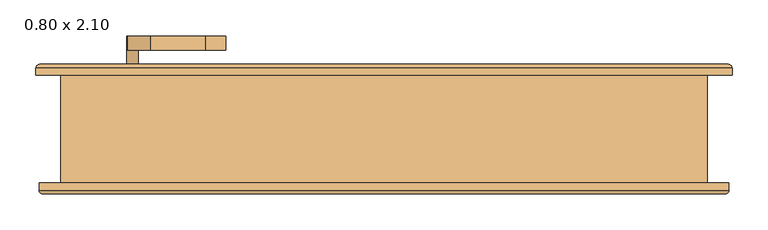
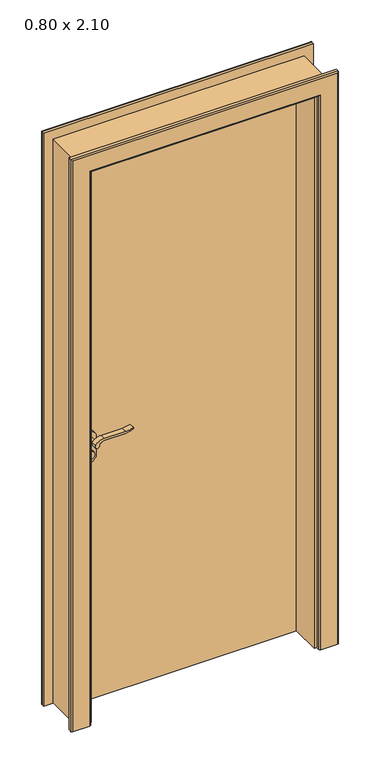
"""IFC4 building model written with IfcOpenShell, lengths in millimetres: door geometry, PORTA_DE_ABRIR_MADEIRA : 0.80 x 2.10."""

from ifc_helpers import new_model, si_unit, point, frame, frame_2d, origin, origin_with_axes, place, context, project, spatial, polyline, circle_curve, ellipse_curve, trimmed, segment, composite_curve, outline, extrude, faceted_brep, source, transform, mapped, element, save
from ifc_brep_helpers import plane_surface, cylinder_surface, advanced_brep


def door_0_80_x_2_10_1ca43dfd(model_context):
    return source(origin(), model_context, "Body", "SolidModel", [
        extrude(outline(composite_curve([segment(trimmed(circle_curve(frame_2d((940.0, -350.0)), 15.0), [point((940.0, -335.0))], [point((940.0, -365.0))], False, "CARTESIAN"), True, "CONTINUOUS"), segment(trimmed(circle_curve(frame_2d((940.0, -350.0)), 15.0), [point((940.0, -365.0))], [point((940.0, -335.0))], False, "CARTESIAN"), True, "CONTINUOUS")], self_intersect=False)), frame((0.0, 15.0, 0.0), z_axis=(0.0, 1.0, 0.0), x_axis=(0.0, 0.0, 1.0)), (0.0, 0.0, 1.0), 10.0),
        extrude(outline(composite_curve([segment(trimmed(circle_curve(frame_2d((940.0, -350.0)), 15.0), [point((940.0, -335.0))], [point((940.0, -365.0))], False, "CARTESIAN"), True, "CONTINUOUS"), segment(trimmed(circle_curve(frame_2d((940.0, -350.0)), 15.0), [point((940.0, -365.0))], [point((940.0, -335.0))], False, "CARTESIAN"), True, "CONTINUOUS")], self_intersect=False)), frame((0.0, 80.0, 0.0), z_axis=(0.0, 1.0, 0.0), x_axis=(0.0, 0.0, 1.0)), (0.0, 0.0, 1.0), 10.0),
        extrude(outline(composite_curve([segment(trimmed(circle_curve(frame_2d((1000.0, -350.0)), 8.0), [point((1004.6523287, -356.5081363))], [point((1000.0, -342.0))], False, "CARTESIAN"), True, "CONTINUOUS"), segment(trimmed(circle_curve(frame_2d((994.8738613, -324.6138099)), 18.1261387), [point((1000.0, -342.0))], [point((1013.0, -324.6138099))], True, "CARTESIAN"), True, "CONTINUOUS"), segment(polyline([(1013.0, -324.6138099), (1013.0, -248.3564091)]), True, "CONTINUOUS"), segment(trimmed(circle_curve(frame_2d((1072.2709207, -251.9396612)), 59.3791355), [point((1013.0, -248.3564091))], [point((1022.2135558, -220.0))], False, "CARTESIAN"), True, "CONTINUOUS"), segment(polyline([(1022.2135558, -220.0), (1025.0, -220.0)]), True, "CONTINUOUS"), segment(trimmed(circle_curve(frame_2d((1103.2850638, -248.4227909)), 83.2850902), [point((1025.0, -220.0))], [point((1020.0, -248.3564091))], True, "CARTESIAN"), True, "CONTINUOUS"), segment(polyline([(1020.0, -248.3564091), (1020.0, -324.6325667)]), True, "CONTINUOUS"), segment(trimmed(circle_curve(frame_2d((982.7555521, -326.3324871)), 37.2832219), [point((1020.0, -324.6325667))], [point((1004.6523287, -356.5081363))], False, "CARTESIAN"), True, "CONTINUOUS")], self_intersect=False)), frame((0.0, -25.0, 0.0), z_axis=(0.0, 1.0, 0.0), x_axis=(0.0, 0.0, 1.0)), (0.0, 0.0, 1.0), 20.0),
        extrude(outline(composite_curve([segment(trimmed(circle_curve(frame_2d((994.8738682, -324.6138122)), 18.1261318), [point((999.9999903, -342.0))], [point((1013.0, -324.6138122))], True, "CARTESIAN"), True, "CONTINUOUS"), segment(polyline([(1013.0, -324.6138122), (1013.0, -248.3564091)]), True, "CONTINUOUS"), segment(trimmed(circle_curve(frame_2d((1072.2709207, -251.9396612)), 59.3791355), [point((1013.0, -248.3564091))], [point((1022.2135558, -220.0))], False, "CARTESIAN"), True, "CONTINUOUS"), segment(polyline([(1022.2135558, -220.0), (1025.0, -220.0)]), True, "CONTINUOUS"), segment(trimmed(circle_curve(frame_2d((1103.2850638, -248.4227909)), 83.2850902), [point((1025.0, -220.0))], [point((1020.0, -248.3564091))], True, "CARTESIAN"), True, "CONTINUOUS"), segment(polyline([(1020.0, -248.3564091), (1020.0, -324.6325667)]), True, "CONTINUOUS"), segment(trimmed(circle_curve(frame_2d((982.7555521, -326.3324871)), 37.2832219), [point((1020.0, -324.6325667))], [point((1004.6523287, -356.5081363))], False, "CARTESIAN"), True, "CONTINUOUS"), segment(trimmed(circle_curve(frame_2d((1000.0, -350.0)), 8.0), [point((1004.6523287, -356.5081363))], [point((999.9999903, -342.0))], False, "CARTESIAN"), True, "CONTINUOUS")], self_intersect=False)), frame((0.0, 110.0, 0.0), z_axis=(0.0, 1.0, 0.0), x_axis=(0.0, 0.0, 1.0)), (0.0, 0.0, 1.0), 20.0),
        extrude(outline(composite_curve([segment(trimmed(circle_curve(frame_2d((1000.0, -350.0)), 8.0), [point((1000.0, -342.0))], [point((1000.0, -358.0))], False, "CARTESIAN"), True, "CONTINUOUS"), segment(trimmed(circle_curve(frame_2d((1000.0, -350.0)), 8.0), [point((1000.0, -358.0))], [point((1000.0, -342.0))], False, "CARTESIAN"), True, "CONTINUOUS")], self_intersect=False)), frame((0.0, -5.0, 0.0), z_axis=(0.0, 1.0, 0.0), x_axis=(0.0, 0.0, 1.0)), (0.0, 0.0, 1.0), 30.0),
        extrude(outline(composite_curve([segment(trimmed(circle_curve(frame_2d((1000.0, -350.0)), 8.0), [point((1000.0, -342.0))], [point((1000.0, -358.0))], False, "CARTESIAN"), True, "CONTINUOUS"), segment(trimmed(circle_curve(frame_2d((1000.0, -350.0)), 8.0), [point((1000.0, -358.0))], [point((1000.0, -342.0))], False, "CARTESIAN"), True, "CONTINUOUS")], self_intersect=False)), frame((0.0, 80.0, 0.0), z_axis=(0.0, 1.0, 0.0), x_axis=(0.0, 0.0, 1.0)), (0.0, 0.0, 1.0), 30.0),
        extrude(outline(composite_curve([segment(trimmed(circle_curve(frame_2d((930.0, -350.0)), 25.0), [point((930.0, -375.0))], [point((930.0, -325.0))], False, "CARTESIAN"), True, "CONTINUOUS"), segment(polyline([(930.0, -325.0), (1000.0, -325.0)]), True, "CONTINUOUS"), segment(trimmed(circle_curve(frame_2d((1000.0, -350.0)), 25.0), [point((1000.0, -325.0))], [point((1000.0, -375.0))], False, "CARTESIAN"), True, "CONTINUOUS"), segment(polyline([(1000.0, -375.0), (930.0, -375.0)]), True, "CONTINUOUS")], self_intersect=False)), frame((0.0, 25.0, 0.0), z_axis=(0.0, 1.0, 0.0), x_axis=(0.0, 0.0, 1.0)), (0.0, 0.0, 1.0), 10.0),
        extrude(outline(composite_curve([segment(trimmed(circle_curve(frame_2d((930.0, -350.0)), 25.0), [point((930.0, -375.0))], [point((930.0, -325.0))], False, "CARTESIAN"), True, "CONTINUOUS"), segment(polyline([(930.0, -325.0), (1000.0, -325.0)]), True, "CONTINUOUS"), segment(trimmed(circle_curve(frame_2d((1000.0, -350.0)), 25.0), [point((1000.0, -325.0))], [point((1000.0, -375.0))], False, "CARTESIAN"), True, "CONTINUOUS"), segment(polyline([(1000.0, -375.0), (930.0, -375.0)]), True, "CONTINUOUS")], self_intersect=False)), frame((0.0, 70.0, 0.0), z_axis=(0.0, 1.0, 0.0), x_axis=(0.0, 0.0, 1.0)), (0.0, 0.0, 1.0), 10.0),
        faceted_brep([(-410.0, 35.0, 0.0), (-400.0, 35.0, 0.0), (-400.0, -75.0, 0.0), (-450.0, -75.0, 0.0), (-450.0, 75.0, 0.0), (-410.0, 75.0, 0.0), (-410.0, 75.0, 2100.0), (-410.0, 35.0, 2100.0), (-450.0, 75.0, 2140.0), (450.0, 75.0, 2140.0), (450.0, 75.0, 0.0), (410.0, 75.0, 0.0), (410.0, 75.0, 2100.0), (-450.0, -75.0, 2140.0), (-400.0, -75.0, 2090.0), (400.0, -75.0, 2090.0), (400.0, -75.0, 0.0), (450.0, -75.0, 0.0), (450.0, -75.0, 2140.0), (-400.0, 35.0, 2090.0), (410.0, 35.0, 2100.0), (410.0, 35.0, 0.0), (400.0, 35.0, 0.0), (400.0, 35.0, 2090.0)], [[[0, 1, 2, 3, 4, 5]], [[5, 6, 7, 0]], [[4, 8, 9, 10, 11, 12, 6, 5]], [[3, 13, 8, 4]], [[2, 14, 15, 16, 17, 18, 13, 3]], [[1, 19, 14, 2]], [[0, 7, 20, 21, 22, 23, 19, 1]], [[23, 22, 16, 15]], [[21, 11, 10, 17, 16, 22]], [[12, 11, 21, 20]], [[18, 17, 10, 9]], [[13, 18, 9, 8]], [[19, 23, 15, 14]], [[6, 12, 20, 7]]]),
        advanced_brep(
        [(-480.0, -75.3, 0.0), (-410.0, -75.3, 0.0), (-410.0, -85.3, 0.0), (-415.0, -90.3, 0.0), (-475.0, -90.3, 0.0), (-480.0, -85.3, 0.0), (-480.0, -85.3, 2170.0), (-480.0, -75.3, 2170.0), (-475.0, -90.3, 2165.0), (-415.0, -90.3, 2105.0), (415.0, -90.3, 2105.0), (415.0, -90.3, 0.0), (475.0, -90.3, 0.0), (475.0, -90.3, 2165.0), (-410.0, -85.3, 2100.0), (-410.0, -75.3, 2100.0), (480.0, -75.3, 2170.0), (480.0, -75.3, 0.0), (410.0, -75.3, 0.0), (410.0, -75.3, 2100.0), (480.0, -85.3, 0.0), (410.0, -85.3, 0.0), (410.0, -85.3, 2100.0), (480.0, -85.3, 2170.0)],
        [
            (0, 1),
            (1, 2),
            (2, 3, circle_curve(frame((-415.0, -85.3, 0.0), z_axis=(0.0, 0.0, -1.0), x_axis=(-1.0, 0.0, 0.0)), 5.0)),
            (3, 4),
            (4, 5, circle_curve(frame((-475.0, -85.3, 0.0), z_axis=(0.0, 0.0, -1.0), x_axis=(-1.0, 0.0, 0.0)), 5.0)),
            (5, 0),
            (5, 6),
            (6, 7),
            (7, 0),
            (4, 8),
            (8, 6, ellipse_curve(frame((-475.0, -85.3, 2165.0), z_axis=(-0.7071067811865475, 0.0, -0.7071067811865475), x_axis=(0.7071067811865474, 0.0, -0.7071067811865476)), 7.0710678, 5.0)),
            (3, 9),
            (9, 10),
            (10, 11),
            (11, 12),
            (12, 13),
            (13, 8),
            (2, 14),
            (14, 9, ellipse_curve(frame((-415.0, -85.3, 2105.0), z_axis=(-0.7071067811865475, 0.0, -0.7071067811865475), x_axis=(0.7071067811865474, 0.0, -0.7071067811865476)), 7.0710678, 5.0)),
            (1, 15),
            (15, 14),
            (7, 16),
            (16, 17),
            (17, 18),
            (18, 19),
            (19, 15),
            (17, 20),
            (20, 12, circle_curve(frame((475.0, -85.3, 0.0), z_axis=(0.0, 0.0, -1.0), x_axis=(1.0, 0.0, 0.0)), 5.0)),
            (11, 21, circle_curve(frame((415.0, -85.3, 0.0), z_axis=(0.0, 0.0, -1.0), x_axis=(1.0, 0.0, 0.0)), 5.0)),
            (21, 18),
            (21, 22),
            (22, 19),
            (10, 22, ellipse_curve(frame((415.0, -85.3, 2105.0), z_axis=(0.7071067811865475, 0.0, -0.7071067811865475), x_axis=(0.7071067811865474, 0.0, 0.7071067811865476)), 7.0710678, 5.0)),
            (20, 23),
            (23, 13, ellipse_curve(frame((475.0, -85.3, 2165.0), z_axis=(0.7071067811865475, 0.0, -0.7071067811865475), x_axis=(0.7071067811865474, 0.0, 0.7071067811865476)), 7.0710678, 5.0)),
            (16, 23),
            (6, 23),
            (22, 14),
        ],
        [
            plane_surface(frame((-450.0, 75.0, 0.0), z_axis=(0.0, 0.0, -1.0), x_axis=(0.0, 1.0, 0.0))),
            plane_surface(frame((-480.0, -75.3, 0.0), z_axis=(-1.0, 0.0, 0.0), x_axis=(0.0, 0.0, 1.0))),
            cylinder_surface(frame((-475.0, -85.3, 0.0), z_axis=(0.0, 0.0, -1.0), x_axis=(-1.0, 0.0, 0.0)), 5.0),
            plane_surface(frame((-475.0, -90.3, 0.0), z_axis=(0.0, -1.0, 0.0), x_axis=(0.0, 0.0, 1.0))),
            cylinder_surface(frame((-415.0, -85.3, 0.0), z_axis=(0.0, 0.0, -1.0), x_axis=(-1.0, 0.0, 0.0)), 5.0),
            plane_surface(frame((-410.0, -85.3, 0.0), z_axis=(1.0, 0.0, 0.0), x_axis=(0.0, 0.0, 1.0))),
            plane_surface(frame((-410.0, -75.3, 0.0), z_axis=(0.0, 1.0, 0.0), x_axis=(0.0, 0.0, 1.0))),
            plane_surface(frame((450.0, 75.0, 0.0), z_axis=(0.0, 0.0, -1.0), x_axis=(0.0, 1.0, 0.0))),
            plane_surface(frame((410.0, -85.3, 2100.0), z_axis=(-1.0, 0.0, 0.0), x_axis=(0.0, 0.0, -1.0))),
            cylinder_surface(frame((415.0, -85.3, 2140.0), z_axis=(0.0, 0.0, 1.0), x_axis=(1.0, 0.0, 0.0)), 5.0),
            cylinder_surface(frame((475.0, -85.3, 2140.0), z_axis=(0.0, 0.0, 1.0), x_axis=(1.0, 0.0, 0.0)), 5.0),
            plane_surface(frame((480.0, -75.3, 2170.0), z_axis=(1.0, 0.0, 0.0), x_axis=(0.0, 0.0, -1.0))),
            plane_surface(frame((-480.0, -75.3, 2170.0), z_axis=(0.0, 0.0, 1.0), x_axis=(1.0, 0.0, 0.0))),
            plane_surface(frame((-410.0, -85.3, 2100.0), z_axis=(0.0, 0.0, -1.0), x_axis=(1.0, 0.0, 0.0))),
            cylinder_surface(frame((-450.0, -85.3, 2165.0), z_axis=(-1.0, 0.0, 0.0), x_axis=(0.0, 0.0, 1.0)), 5.0),
            cylinder_surface(frame((-450.0, -85.3, 2105.0), z_axis=(-1.0, 0.0, 0.0), x_axis=(0.0, 0.0, 1.0)), 5.0),
        ],
        [
            (0, [[1, 2, 3, 4, 5, 6]]),
            (1, [[7, 8, 9, -6]]),
            (2, [[10, 11, -7, -5]]),
            (3, [[12, 13, 14, 15, 16, 17, -10, -4]]),
            (4, [[18, 19, -12, -3]]),
            (5, [[20, 21, -18, -2]]),
            (6, [[-9, 22, 23, 24, 25, 26, -20, -1]]),
            (7, [[27, 28, -15, 29, 30, -24]]),
            (8, [[-25, -30, 31, 32]]),
            (9, [[-31, -29, -14, 33]]),
            (10, [[-16, -28, 34, 35]]),
            (11, [[-34, -27, -23, 36]]),
            (12, [[37, -36, -22, -8]]),
            (13, [[-26, -32, 38, -21]]),
            (14, [[-17, -35, -37, -11]]),
            (15, [[-38, -33, -13, -19]]),
        ],
    ),
        advanced_brep(
        [(-479.3155593, 90.2647517, 0.0), (-419.3155593, 90.2647517, 0.0), (-414.3155593, 85.2647517, 0.0), (-414.3155593, 75.2647517, 0.0), (-484.3155593, 75.2647517, 0.0), (-484.3155593, 85.2647517, 0.0), (-484.3155593, 85.2647517, 2174.3155593), (-479.3155593, 90.2647517, 2169.3155593), (-484.3155593, 75.2647517, 2174.3155593), (-414.3155593, 75.2647517, 2104.3155593), (414.3155593, 75.2647517, 2104.3155593), (414.3155593, 75.2647517, 0.0), (484.3155593, 75.2647517, 0.0), (484.3155593, 75.2647517, 2174.3155593), (-414.3155593, 85.2647517, 2104.3155593), (-419.3155593, 90.2647517, 2109.3155593), (479.3155593, 90.2647517, 2169.3155593), (479.3155593, 90.2647517, 0.0), (419.3155593, 90.2647517, 0.0), (419.3155593, 90.2647517, 2109.3155593), (484.3155593, 85.2647517, 0.0), (414.3155593, 85.2647517, 0.0), (414.3155593, 85.2647517, 2104.3155593), (484.3155593, 85.2647517, 2174.3155593)],
        [
            (0, 1),
            (1, 2, circle_curve(frame((-419.3155593, 85.2647517, 0.0), z_axis=(0.0, 0.0, -1.0), x_axis=(-1.0, 0.0, 0.0)), 5.0)),
            (2, 3),
            (3, 4),
            (4, 5),
            (5, 0, circle_curve(frame((-479.3155593, 85.2647517, 0.0), z_axis=(0.0, 0.0, -1.0), x_axis=(-1.0, 0.0, 0.0)), 5.0)),
            (5, 6),
            (6, 7, ellipse_curve(frame((-479.3155593, 85.2647517, 2169.3155593), z_axis=(-0.7071067811865475, 0.0, -0.7071067811865475), x_axis=(0.7071067811865474, 0.0, -0.7071067811865476)), 7.0710678, 5.0)),
            (7, 0),
            (4, 8),
            (8, 6),
            (3, 9),
            (9, 10),
            (10, 11),
            (11, 12),
            (12, 13),
            (13, 8),
            (2, 14),
            (14, 9),
            (1, 15),
            (15, 14, ellipse_curve(frame((-419.3155593, 85.2647517, 2109.3155593), z_axis=(-0.7071067811865475, 0.0, -0.7071067811865475), x_axis=(0.7071067811865474, 0.0, -0.7071067811865476)), 7.0710678, 5.0)),
            (7, 16),
            (16, 17),
            (17, 18),
            (18, 19),
            (19, 15),
            (17, 20, circle_curve(frame((479.3155593, 85.2647517, 0.0), z_axis=(0.0, 0.0, -1.0), x_axis=(1.0, 0.0, 0.0)), 5.0)),
            (20, 12),
            (11, 21),
            (21, 18, circle_curve(frame((419.3155593, 85.2647517, 0.0), z_axis=(0.0, 0.0, -1.0), x_axis=(1.0, 0.0, 0.0)), 5.0)),
            (21, 22),
            (22, 19, ellipse_curve(frame((419.3155593, 85.2647517, 2109.3155593), z_axis=(0.7071067811865475, 0.0, -0.7071067811865475), x_axis=(0.7071067811865474, 0.0, 0.7071067811865476)), 7.0710678, 5.0)),
            (10, 22),
            (20, 23),
            (23, 13),
            (16, 23, ellipse_curve(frame((479.3155593, 85.2647517, 2169.3155593), z_axis=(0.7071067811865475, 0.0, -0.7071067811865475), x_axis=(0.7071067811865474, 0.0, 0.7071067811865476)), 7.0710678, 5.0)),
            (23, 6),
            (14, 22),
        ],
        [
            plane_surface(frame((-450.0, 75.0, 0.0), z_axis=(0.0, 0.0, -1.0), x_axis=(0.0, 1.0, 0.0))),
            cylinder_surface(frame((-479.3155593, 85.2647517, 0.0), z_axis=(0.0, 0.0, -1.0), x_axis=(-1.0, 0.0, 0.0)), 5.0),
            plane_surface(frame((-484.3155593, 85.2647517, 0.0), z_axis=(-1.0, 0.0, 0.0), x_axis=(0.0, 0.0, 1.0))),
            plane_surface(frame((-484.3155593, 75.2647517, 0.0), z_axis=(0.0, -1.0, 0.0), x_axis=(0.0, 0.0, 1.0))),
            plane_surface(frame((-414.3155593, 75.2647517, 0.0), z_axis=(1.0, 0.0, 0.0), x_axis=(0.0, 0.0, 1.0))),
            cylinder_surface(frame((-419.3155593, 85.2647517, 0.0), z_axis=(0.0, 0.0, -1.0), x_axis=(-1.0, 0.0, 0.0)), 5.0),
            plane_surface(frame((-419.3155593, 90.2647517, 0.0), z_axis=(0.0, 1.0, 0.0), x_axis=(0.0, 0.0, 1.0))),
            plane_surface(frame((450.0, 75.0, 0.0), z_axis=(0.0, 0.0, -1.0), x_axis=(0.0, 1.0, 0.0))),
            cylinder_surface(frame((419.3155593, 85.2647517, 2140.0), z_axis=(0.0, 0.0, 1.0), x_axis=(1.0, 0.0, 0.0)), 5.0),
            plane_surface(frame((414.3155593, 75.2647517, 2104.3155593), z_axis=(-1.0, 0.0, 0.0), x_axis=(0.0, 0.0, -1.0))),
            plane_surface(frame((484.3155593, 85.2647517, 2174.3155593), z_axis=(1.0, 0.0, 0.0), x_axis=(0.0, 0.0, -1.0))),
            cylinder_surface(frame((479.3155593, 85.2647517, 2140.0), z_axis=(0.0, 0.0, 1.0), x_axis=(1.0, 0.0, 0.0)), 5.0),
            plane_surface(frame((-484.3155593, 85.2647517, 2174.3155593), z_axis=(0.0, 0.0, 1.0), x_axis=(1.0, 0.0, 0.0))),
            plane_surface(frame((-414.3155593, 75.2647517, 2104.3155593), z_axis=(0.0, 0.0, -1.0), x_axis=(1.0, 0.0, 0.0))),
            cylinder_surface(frame((-450.0, 85.2647517, 2169.3155593), z_axis=(-1.0, 0.0, 0.0), x_axis=(0.0, 0.0, 1.0)), 5.0),
            cylinder_surface(frame((-450.0, 85.2647517, 2109.3155593), z_axis=(-1.0, 0.0, 0.0), x_axis=(0.0, 0.0, 1.0)), 5.0),
        ],
        [
            (0, [[1, 2, 3, 4, 5, 6]]),
            (1, [[7, 8, 9, -6]]),
            (2, [[10, 11, -7, -5]]),
            (3, [[12, 13, 14, 15, 16, 17, -10, -4]]),
            (4, [[18, 19, -12, -3]]),
            (5, [[20, 21, -18, -2]]),
            (6, [[-9, 22, 23, 24, 25, 26, -20, -1]]),
            (7, [[27, 28, -15, 29, 30, -24]]),
            (8, [[-25, -30, 31, 32]]),
            (9, [[-31, -29, -14, 33]]),
            (10, [[-16, -28, 34, 35]]),
            (11, [[-34, -27, -23, 36]]),
            (12, [[-17, -35, 37, -11]]),
            (13, [[38, -33, -13, -19]]),
            (14, [[-37, -36, -22, -8]]),
            (15, [[-26, -32, -38, -21]]),
        ],
    ),
        extrude(outline(polyline([(410.0, 70.0), (410.0, 35.0), (-410.0, 35.0), (-410.0, 70.0), (410.0, 70.0)])), origin_with_axes(), (0.0, 0.0, 1.0), 2100.0),
    ])


if __name__ == "__main__":
    model = new_model("IFC4")
    model_context = context("Model", 3, world=origin())
    ifc_project = project(units=[si_unit("LENGTHUNIT", "METRE", prefix="MILLI")], contexts=[model_context])
    site = spatial("IfcSite", under=ifc_project)
    building = spatial("IfcBuilding", under=site)
    placement = place(None, origin())
    door_0_80_x_2_10_shape = door_0_80_x_2_10_1ca43dfd(model_context)
    element("IfcDoor", 1, ObjectType="PORTA_DE_ABRIR_MADEIRA : 0.80 x 2.10", at=placement, inside=building, context=model_context, shape_type="MappedRepresentation", body=[
        mapped(door_0_80_x_2_10_shape, transform((0.0, 0.0, 0.0), x_axis=(1.0, 0.0, 0.0), y_axis=(0.0, 1.0, 0.0), z_axis=(0.0, 0.0, 1.0))),
    ])
    save(model, "model.ifc")

# Revit data of these elements
# Type "PORTA_DE_ABRIR_MADEIRA : 0.80 x 2.10"
#   Type Mark = "P2"
#   Analytic Construction = "<Nenhum>"
#   Rough Width = 0.90 m
#   Projeção da estrutura externa = 0.50 m
#   Projeção da estrutura interna = 0.025 m
#   Largura da estrutura = 0.075 m
#   Rough Height = 2.15 m
#   Height = 2.10 m
#   Width = 0.80 m
#   Soleira [instance default] = no
#   Material do batente = .BATENTE E GUARNIÇÃO
#   Material da maçaneta = .AÇO INOXIDÁVEL ESCOVADO
#   Material da folha da porta = .FOLHA DA PORTA
#   Material da Soleira [instance default] = none
#   Function = (empty or 0)
#   Wall Closure = (empty or 0)
# Element 1 (IfcDoor, "PORTA_DE_ABRIR_MADEIRA : 0.80 x 2.10")
#   Materials on its faces: ".AÇO INOXIDÁVEL ESCOVADO", ".BATENTE E GUARNIÇÃO", ".FOLHA DA PORTA"
# Materials
#   ".BATENTE E GUARNIÇÃO": class "Madeira", colour RGB 215 186 156, transparency 0, Cost = 0
#   ".AÇO INOXIDÁVEL ESCOVADO": class "Metal", colour RGB 189 187 185, transparency 0, Description = "Stainless Steel 18/8, brushed finish", Cost = 0
#   ".FOLHA DA PORTA": class "Madeira", colour RGB 148 119 91, transparency 0, Cost = 0
